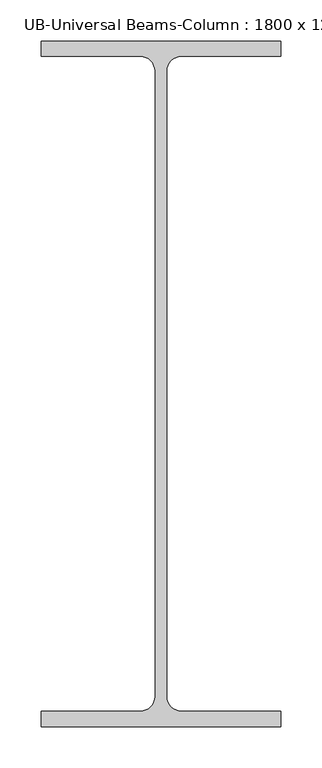
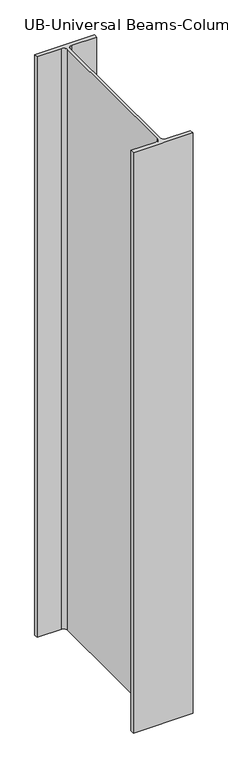
"""IFC4 building model written with IfcOpenShell, lengths in millimetres: column geometry, UB-Universal Beams-Column : 1800 x 1200 x 450mm."""

from ifc_helpers import new_model, si_unit, point, frame_2d, origin, origin_with_axes, place, context, project, spatial, polyline, circle_curve, trimmed, segment, composite_curve, outline, extrude, source, transform, mapped, element, save


def ub_universal_beams_column_1800_x_1200_x_450mm_b070674e(model_context):
    return source(origin(), model_context, "Body", "SweptSolid", [
        extrude(outline(composite_curve([segment(polyline([(145.85, 417.45), (145.85, 398.65), (24.8, 398.65)]), True, "CONTINUOUS"), segment(trimmed(circle_curve(frame_2d((24.8, 380.85)), 17.8), [point((24.8, 398.65))], [point((7.0, 380.85))], True, "CARTESIAN"), True, "CONTINUOUS"), segment(polyline([(7.0, 380.85), (7.0, -380.85)]), True, "CONTINUOUS"), segment(trimmed(circle_curve(frame_2d((24.8, -380.85)), 17.8), [point((7.0, -380.85))], [point((24.8, -398.65))], True, "CARTESIAN"), True, "CONTINUOUS"), segment(polyline([(24.8, -398.65), (145.85, -398.65), (145.85, -417.45), (-145.85, -417.45), (-145.85, -398.65), (-24.8, -398.65)]), True, "CONTINUOUS"), segment(trimmed(circle_curve(frame_2d((-24.8, -380.85)), 17.8), [point((-24.8, -398.65))], [point((-7.0, -380.85))], True, "CARTESIAN"), True, "CONTINUOUS"), segment(polyline([(-7.0, -380.85), (-7.0, 380.85)]), True, "CONTINUOUS"), segment(trimmed(circle_curve(frame_2d((-24.8, 380.85)), 17.8), [point((-7.0, 380.85))], [point((-24.8, 398.65))], True, "CARTESIAN"), True, "CONTINUOUS"), segment(polyline([(-24.8, 398.65), (-145.85, 398.65), (-145.85, 417.45), (145.85, 417.45)]), True, "CONTINUOUS")], self_intersect=False)), origin_with_axes(), (0.0, 0.0, 1.0), 3000.0),
    ])


if __name__ == "__main__":
    model = new_model("IFC4")
    model_context = context("Model", 3, world=origin())
    ifc_project = project(units=[si_unit("LENGTHUNIT", "METRE", prefix="MILLI")], contexts=[model_context])
    site = spatial("IfcSite", under=ifc_project)
    building = spatial("IfcBuilding", under=site)
    placement = place(None, origin())
    ub_universal_beams_column_1800_x_1200_x_450mm_shape = ub_universal_beams_column_1800_x_1200_x_450mm_b070674e(model_context)
    element("IfcColumn", 1, ObjectType="UB-Universal Beams-Column : 1800 x 1200 x 450mm", at=placement, inside=building, context=model_context, shape_type="MappedRepresentation", body=[
        mapped(ub_universal_beams_column_1800_x_1200_x_450mm_shape, transform((0.0, 0.0, 0.0), x_axis=(1.0, 0.0, 0.0), y_axis=(0.0, 1.0, 0.0), z_axis=(0.0, 0.0, 1.0))),
    ])
    save(model, "model.ifc")

# Revit data of these elements
# Type "UB-Universal Beams-Column : 1800 x 1200 x 450mm"
#   Section Name Key = "UB838x292x176"
#   Width = 29.17 cm
#   Web Thickness = 1.4 cm
#   Web Fillet = 1.78 cm
#   Warping Constant = 13000000.0 cm⁶
#   Torsional Moment of Inertia = 221.00 cm⁴
#   Section Area = 224.0 cm²
#   Plastic Modulus weak axis = 842.0 cm³
#   Plastic Modulus strong axis = 6808.0 cm³
#   Nominal Weight = 175.899 kgf/m
#   Moment of Inertia weak axis = 7799.00 cm⁴
#   Moment of Inertia strong axis = 246021.00 cm⁴
#   Height = 83.49 cm
#   Flange Thickness = 1.88 cm
#   Elastic Modulus weak axis = 535.0 cm³
#   Elastic Modulus strong axis = 5893.0 cm³
#   Centroid Vertical = 41.745 cm
#   Centroid Horizontal = 14.585 cm
#   Bolt Spacing = 14.0 cm
#   Structural Material [instance default] = Metal - Steel 43-275
#   Type Comments = ""
#   Assembly Code = ""
# Element 1 (IfcColumn, "UB-Universal Beams-Column : 1800 x 1200 x 450mm")
#   Materials on its faces: "Metal - Steel 43-275"
# Materials
#   "Metal - Steel 43-275": class "Metal", colour RGB 247 247 247, transparency 0, Cost = 0
